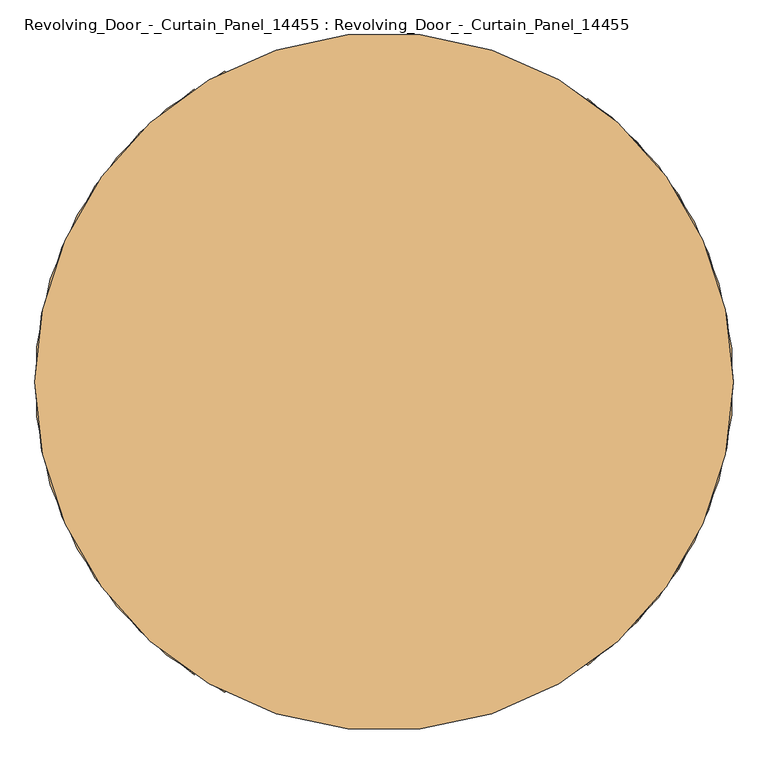
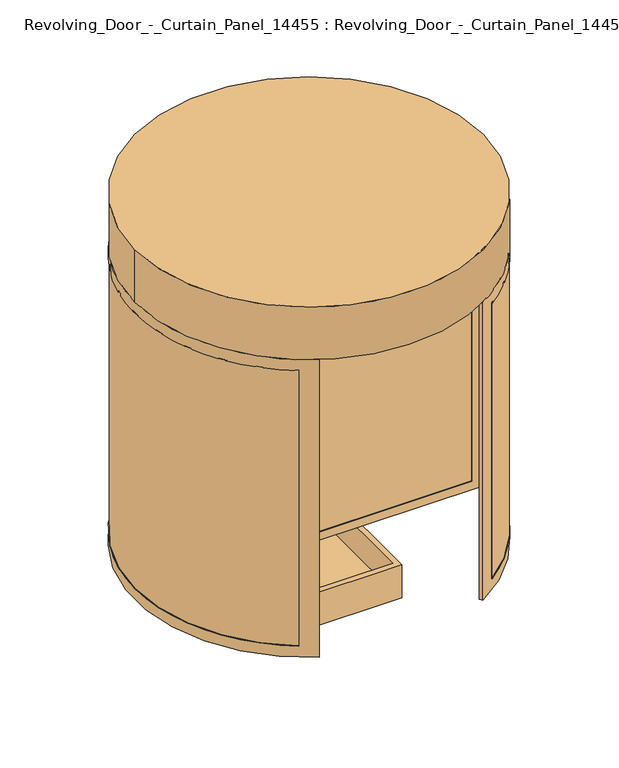
"""IFC4 building model written with IfcOpenShell, lengths in millimetres: door geometry, Revolving_Door_-_Curtain_Panel_14455 : Revolving_Door_-_Curtain_Panel_14455."""

from ifc_helpers import new_model, si_unit, point, frame, origin, origin_with_axes, origin_2d, place, context, project, spatial, polyline, circle_curve, trimmed, segment, composite_curve, outline, extrude, faceted_brep, source, transform, mapped, element, save
from ifc_brep_helpers import plane_surface, cylinder_surface, revolved_surface, advanced_brep


def revolving_door_curtain_panel_14455_revolving_door_curtain_311cc346(model_context):
    return source(origin(), model_context, "Body", "SolidModel", [
        extrude(outline(composite_curve([segment(trimmed(circle_curve(origin_2d(), 1480.0), [point((-804.0011256, -1242.5707988))], [point((-804.0011256, 1242.5707988))], False, "CARTESIAN"), True, "CONTINUOUS"), segment(polyline([(-804.0011256, 1242.5707988), (-793.9880841, 1225.2277022)]), True, "CONTINUOUS"), segment(trimmed(circle_curve(origin_2d(), 1460.0), [point((-793.9880841, 1225.2277022))], [point((-793.9880841, -1225.2277022))], True, "CARTESIAN"), True, "CONTINUOUS"), segment(polyline([(-793.9880841, -1225.2277022), (-804.0011256, -1242.5707988)]), True, "CONTINUOUS")], self_intersect=False)), frame((0.0, 0.0, 100.0), z_axis=(0.0, 0.0, 1.0), x_axis=(1.0, 0.0, 0.0)), (0.0, 0.0, 1.0), 2485.0),
        extrude(outline(composite_curve([segment(polyline([(863.2115619, -1202.1920809), (853.1615488, -1184.7849474)]), True, "CONTINUOUS"), segment(trimmed(circle_curve(origin_2d(), 1460.0), [point((853.1615488, -1184.7849474))], [point((853.1615488, 1184.7849474))], True, "CARTESIAN"), True, "CONTINUOUS"), segment(polyline([(853.1615488, 1184.7849474), (863.2115619, 1202.1920809)]), True, "CONTINUOUS"), segment(trimmed(circle_curve(origin_2d(), 1480.0), [point((863.2115619, 1202.1920809))], [point((863.2115619, -1202.1920809))], False, "CARTESIAN"), True, "CONTINUOUS")], self_intersect=False)), frame((0.0, 0.0, 100.0), z_axis=(0.0, 0.0, 1.0), x_axis=(1.0, 0.0, 0.0)), (0.0, 0.0, 1.0), 2485.0),
        advanced_brep(
        [(-676.6005204, -1321.9064777, 0.0), (-676.6005204, 1321.9064777, 0.0), (-661.580957, 1295.8918309, 0.0), (-661.580957, -1295.8918309, 0.0), (-676.6005204, -1321.9064777, 2685.0), (-661.580957, -1295.8918309, 2685.0), (-661.580957, 1295.8918309, 2685.0), (-791.4847676, 1220.8918309, 2585.0), (-791.4847676, 1220.8918309, 100.0), (-791.4847676, -1220.8918309, 100.0), (-791.4847676, -1220.8918309, 2585.0), (-676.6005204, 1321.9064777, 2685.0), (-806.5043309, -1246.9064777, 2585.0), (-806.5043309, -1246.9064777, 100.0), (-806.5043309, 1246.9064777, 100.0), (-806.5043309, 1246.9064777, 2585.0)],
        [
            (0, 1, circle_curve(frame((0.0, 0.0, 0.0), z_axis=(0.0, 0.0, -1.0), x_axis=(1.0, 0.0, 0.0)), 1485.0)),
            (1, 2),
            (2, 3, circle_curve(origin_with_axes(), 1455.0)),
            (3, 0),
            (4, 0),
            (3, 5),
            (5, 4),
            (2, 6),
            (6, 5, circle_curve(frame((0.0, 0.0, 2685.0), z_axis=(0.0, 0.0, 1.0), x_axis=(1.0, 0.0, 0.0)), 1455.0)),
            (7, 8),
            (8, 9, circle_curve(frame((0.0, 0.0, 100.0), z_axis=(0.0, 0.0, 1.0), x_axis=(1.0, 0.0, 0.0)), 1455.0)),
            (9, 10),
            (10, 7, circle_curve(frame((0.0, 0.0, 2585.0), z_axis=(0.0, 0.0, -1.0), x_axis=(1.0, 0.0, 0.0)), 1455.0)),
            (1, 11),
            (11, 6),
            (4, 11, circle_curve(frame((0.0, 0.0, 2685.0), z_axis=(0.0, 0.0, -1.0), x_axis=(1.0, 0.0, 0.0)), 1485.0)),
            (12, 13),
            (13, 14, circle_curve(frame((0.0, 0.0, 100.0), z_axis=(0.0, 0.0, -1.0), x_axis=(1.0, 0.0, 0.0)), 1485.0)),
            (14, 15),
            (15, 12, circle_curve(frame((0.0, 0.0, 2585.0), z_axis=(0.0, 0.0, 1.0), x_axis=(1.0, 0.0, 0.0)), 1485.0)),
            (14, 8),
            (7, 15),
            (13, 9),
            (12, 10),
        ],
        [
            plane_surface(frame((1485.0, 0.0, 0.0), z_axis=(0.0, 0.0, -1.0), x_axis=(0.0, 1.0, 0.0))),
            plane_surface(frame((-661.580957, -1295.8918309, 2685.0), z_axis=(0.8660254037853362, -0.4999999999984455, 0.0), x_axis=(0.0, 0.0, -1.0))),
            revolved_surface(polyline([(1455.0, 0.0, 0.0), (1455.0, 0.0, 2685.0)]), (0.0, 0.0, 0.0), (0.0, 0.0, -1.0)),
            plane_surface(frame((-676.6005204, 1321.9064777, 2685.0), z_axis=(0.8660254037848054, 0.49999999999936495, 0.0), x_axis=(0.0, 0.0, -1.0))),
            cylinder_surface(origin_with_axes(), 1485.0),
            plane_surface(frame((-806.5043309, 1246.9064777, 2585.0), z_axis=(-0.8660254037848982, -0.4999999999992039, 0.0), x_axis=(0.0, 0.0, -1.0))),
            plane_surface(frame((1485.0, 0.0, 100.0), z_axis=(0.0, 0.0, 1.0), x_axis=(0.0, 1.0, 0.0))),
            plane_surface(frame((-791.4847676, -1220.8918309, 2585.0), z_axis=(-0.8660254037853279, 0.4999999999984598, 0.0), x_axis=(0.0, 0.0, -1.0))),
            plane_surface(frame((1485.0, 0.0, 2685.0), z_axis=(0.0, 0.0, 1.0), x_axis=(0.0, -1.0, 0.0))),
            plane_surface(frame((1485.0, 0.0, 2585.0), z_axis=(0.0, 0.0, -1.0), x_axis=(0.0, -1.0, 0.0))),
        ],
        [
            (0, [[1, 2, 3, 4]]),
            (1, [[5, -4, 6, 7]]),
            (2, [[-6, -3, 8, 9], [10, 11, 12, 13]]),
            (3, [[-8, -2, 14, 15]]),
            (4, [[-14, -1, -5, 16], [17, 18, 19, 20]]),
            (5, [[-19, 21, -10, 22]]),
            (6, [[-18, 23, -11, -21]]),
            (7, [[-12, -23, -17, 24]]),
            (8, [[-7, -9, -15, -16]]),
            (9, [[-20, -22, -13, -24]]),
        ],
    ),
        advanced_brep(
        [(739.4383185, -1287.8105346, 0.0), (724.4382752, -1261.8296975, 0.0), (724.4382752, 1261.8296975, 0.0), (739.4383185, 1287.8105346, 0.0), (739.4383185, -1287.8105346, 2685.0), (739.4383185, 1287.8105346, 2685.0), (865.7238532, 1206.5434969, 2585.0), (865.7238532, 1206.5434969, 100.0), (865.7238532, -1206.5434969, 100.0), (865.7238532, -1206.5434969, 2585.0), (724.4382752, 1261.8296975, 2685.0), (724.4382752, -1261.8296975, 2685.0), (850.648829, -1180.4327892, 2585.0), (850.648829, -1180.4327892, 100.0), (850.648829, 1180.4327892, 100.0), (850.648829, 1180.4327892, 2585.0)],
        [
            (0, 1),
            (1, 2, circle_curve(origin_with_axes(), 1455.0)),
            (2, 3),
            (3, 0, circle_curve(frame((0.0, 0.0, 0.0), z_axis=(0.0, 0.0, -1.0), x_axis=(1.0, 0.0, 0.0)), 1485.0)),
            (4, 0),
            (3, 5),
            (5, 4, circle_curve(frame((0.0, 0.0, 2685.0), z_axis=(0.0, 0.0, -1.0), x_axis=(1.0, 0.0, 0.0)), 1485.0)),
            (6, 7),
            (7, 8, circle_curve(frame((0.0, 0.0, 100.0), z_axis=(0.0, 0.0, -1.0), x_axis=(1.0, 0.0, 0.0)), 1485.0)),
            (8, 9),
            (9, 6, circle_curve(frame((0.0, 0.0, 2585.0), z_axis=(0.0, 0.0, 1.0), x_axis=(1.0, 0.0, 0.0)), 1485.0)),
            (2, 10),
            (10, 5),
            (1, 11),
            (11, 10, circle_curve(frame((0.0, 0.0, 2685.0), z_axis=(0.0, 0.0, 1.0), x_axis=(1.0, 0.0, 0.0)), 1455.0)),
            (12, 13),
            (13, 14, circle_curve(frame((0.0, 0.0, 100.0), z_axis=(0.0, 0.0, 1.0), x_axis=(1.0, 0.0, 0.0)), 1455.0)),
            (14, 15),
            (15, 12, circle_curve(frame((0.0, 0.0, 2585.0), z_axis=(0.0, 0.0, -1.0), x_axis=(1.0, 0.0, 0.0)), 1455.0)),
            (4, 11),
            (7, 14),
            (13, 8),
            (6, 15),
            (12, 9),
        ],
        [
            plane_surface(frame((1485.0, 0.0, 0.0), z_axis=(0.0, 0.0, -1.0), x_axis=(0.0, 1.0, 0.0))),
            cylinder_surface(origin_with_axes(), 1485.0),
            plane_surface(frame((724.4382752, 1261.8296975, 2685.0), z_axis=(-0.866025403784442, 0.49999999999999406, 0.0), x_axis=(0.0, 0.0, -1.0))),
            revolved_surface(polyline([(1455.0, 0.0, 0.0), (1455.0, 0.0, 2685.0)]), (0.0, 0.0, 0.0), (0.0, 0.0, -1.0)),
            plane_surface(frame((739.4383185, -1287.8105346, 2685.0), z_axis=(-0.8660254037846041, -0.49999999999971345, 0.0), x_axis=(0.0, 0.0, -1.0))),
            plane_surface(frame((1485.0, 0.0, 100.0), z_axis=(0.0, 0.0, 1.0), x_axis=(0.0, 1.0, 0.0))),
            plane_surface(frame((850.648829, 1180.4327892, 2585.0), z_axis=(0.8660254037844431, -0.4999999999999923, 0.0), x_axis=(0.0, 0.0, -1.0))),
            plane_surface(frame((865.7238532, -1206.5434969, 2585.0), z_axis=(0.8660254037845999, 0.4999999999997206, 0.0), x_axis=(0.0, 0.0, -1.0))),
            plane_surface(frame((1485.0, 0.0, 2685.0), z_axis=(0.0, 0.0, 1.0), x_axis=(0.0, -1.0, 0.0))),
            plane_surface(frame((1485.0, 0.0, 2585.0), z_axis=(0.0, 0.0, -1.0), x_axis=(0.0, -1.0, 0.0))),
        ],
        [
            (0, [[1, 2, 3, 4]]),
            (1, [[5, -4, 6, 7], [8, 9, 10, 11]]),
            (2, [[-6, -3, 12, 13]]),
            (3, [[-12, -2, 14, 15], [16, 17, 18, 19]]),
            (4, [[-14, -1, -5, 20]]),
            (5, [[-9, 21, -17, 22]]),
            (6, [[-18, -21, -8, 23]]),
            (7, [[-10, -22, -16, 24]]),
            (8, [[-7, -13, -15, -20]]),
            (9, [[-11, -24, -19, -23]]),
        ],
    ),
        extrude(outline(polyline([(-9.9410218, 33.2183548), (-23.7974282, 25.2183548), (-676.2974282, 1155.3815067), (-662.4410218, 1163.3815067), (-9.9410218, 33.2183548)])), frame((0.0, 0.0, 75.0), z_axis=(0.0, 0.0, 1.0), x_axis=(1.0, 0.0, 0.0)), (0.0, 0.0, 1.0), 2535.0),
        extrude(outline(polyline([(1455.0, 0.0), (0.0, 0.0), (0.0, 2685.0), (1455.0, 2685.0), (1455.0, 0.0)]), holes=[polyline([(75.0, 2610.0), (75.0, 75.0), (1380.0, 75.0), (1380.0, 2610.0), (75.0, 2610.0)])]), frame((7.640394, -43.2335505, 0.0), z_axis=(0.8660254037844434, 0.4999999999999919, 0.0), x_axis=(-0.4999999999999919, 0.8660254037844434, 0.0)), (0.0, 0.0, 1.0), 30.0),
        extrude(outline(polyline([(-23.7974282, -25.2183548), (-9.9410218, -33.2183548), (-662.4410218, -1163.3815067), (-676.2974282, -1155.3815067), (-23.7974282, -25.2183548)])), frame((0.0, 0.0, 75.0), z_axis=(0.0, 0.0, 1.0), x_axis=(1.0, 0.0, 0.0)), (0.0, 0.0, 1.0), 2535.0),
        extrude(outline(polyline([(1455.0, 0.0), (0.0, 0.0), (0.0, 2685.0), (1455.0, 2685.0), (1455.0, 0.0)]), holes=[polyline([(75.0, 2610.0), (75.0, 75.0), (1380.0, 75.0), (1380.0, 2610.0), (75.0, 2610.0)])]), frame((33.6211561, 28.2335505, 0.0), z_axis=(-0.8660254037844325, 0.5000000000000107, 0.0), x_axis=(-0.5000000000000107, -0.8660254037844325, 0.0)), (0.0, 0.0, 1.0), 30.0),
        extrude(outline(polyline([(75.0, -8.0), (75.0, 8.0), (1380.0, 8.0), (1380.0, -8.0), (75.0, -8.0)])), frame((0.0, 0.0, 75.0), z_axis=(0.0, 0.0, 1.0), x_axis=(1.0, 0.0, 0.0)), (0.0, 0.0, 1.0), 2535.0),
        extrude(outline(polyline([(0.0, 0.0), (0.0, 1455.0), (2685.0, 1455.0), (2685.0, 0.0), (0.0, 0.0)]), holes=[polyline([(2610.0, 1380.0), (75.0, 1380.0), (75.0, 75.0), (2610.0, 75.0), (2610.0, 1380.0)])]), frame((0.0, -15.0, 0.0), z_axis=(0.0, 1.0, 0.0), x_axis=(0.0, 0.0, 1.0)), (0.0, 0.0, 1.0), 30.0),
        extrude(outline(composite_curve([segment(trimmed(circle_curve(origin_2d(), 50.0), [point((-50.0, 0.0))], [point((50.0, 0.0))], False, "CARTESIAN"), True, "CONTINUOUS"), segment(trimmed(circle_curve(origin_2d(), 50.0), [point((50.0, 0.0))], [point((-50.0, 0.0))], False, "CARTESIAN"), True, "CONTINUOUS")], self_intersect=False)), origin_with_axes(), (0.0, 0.0, 1.0), 2685.0),
        extrude(outline(composite_curve([segment(trimmed(circle_curve(origin_2d(), 1485.0), [point((-1485.0, 0.0))], [point((1485.0, 0.0))], False, "CARTESIAN"), True, "CONTINUOUS"), segment(trimmed(circle_curve(origin_2d(), 1485.0), [point((1485.0, 0.0))], [point((-1485.0, 0.0))], False, "CARTESIAN"), True, "CONTINUOUS")], self_intersect=False)), frame((0.0, 0.0, 2685.0), z_axis=(0.0, 0.0, 1.0), x_axis=(1.0, 0.0, 0.0)), (0.0, 0.0, 1.0), 475.0),
        faceted_brep([(400.0, -542.9342021, -250.0), (400.0, 400.0, -250.0), (-400.0, 400.0, -250.0), (-400.0, -542.9342021, -250.0), (450.0, 450.0, -300.0), (450.0, -592.9342021, -300.0), (-450.0, -592.9342021, -300.0), (-450.0, 450.0, -300.0), (450.0, 450.0, 0.0), (450.0, -592.9342021, 0.0), (-450.0, -592.9342021, 0.0), (-450.0, 450.0, 0.0), (-400.0, -542.9342021, 0.0), (-400.0, 400.0, 0.0), (400.0, 400.0, 0.0), (400.0, -542.9342021, 0.0)], [[[0, 1, 2, 3]], [[4, 5, 6, 7]], [[4, 8, 9, 5]], [[9, 10, 6, 5]], [[10, 11, 7, 6]], [[11, 8, 4, 7]], [[8, 11, 10, 9], [12, 13, 14, 15]], [[15, 0, 3, 12]], [[14, 1, 0, 15]], [[13, 2, 1, 14]], [[12, 3, 2, 13]]]),
    ])


if __name__ == "__main__":
    model = new_model("IFC4")
    model_context = context("Model", 3, world=origin())
    ifc_project = project(units=[si_unit("LENGTHUNIT", "METRE", prefix="MILLI")], contexts=[model_context])
    site = spatial("IfcSite", under=ifc_project)
    building = spatial("IfcBuilding", under=site)
    placement = place(None, origin())
    revolving_door_curtain_panel_14455_revolving_door_curtain_shape = revolving_door_curtain_panel_14455_revolving_door_curtain_311cc346(model_context)
    element("IfcDoor", 1, ObjectType="Revolving_Door_-_Curtain_Panel_14455 : Revolving_Door_-_Curtain_Panel_14455", at=placement, inside=building, context=model_context, shape_type="MappedRepresentation", body=[
        mapped(revolving_door_curtain_panel_14455_revolving_door_curtain_shape, transform((0.0, 0.0, 0.0), x_axis=(1.0, 0.0, 0.0), y_axis=(0.0, 1.0, 0.0), z_axis=(0.0, 0.0, 1.0))),
    ])
    save(model, "model.ifc")

# Revit data of these elements
# Type "Revolving_Door_-_Curtain_Panel_14455 : Revolving_Door_-_Curtain_Panel_14455"
#   Model = "55465463453y7"
#   Manufacturer = "Dublin Doors"
#   Description = "Revolving Door"
#   Type Mark = "42"
#   Fire Rating = "30M"
#   COBie.Type.CreatedBy = "design@eagle.com"
#   COBie.Type.CreatedOn = "2016-09-13T05:47:35"
#   COBie.Type.Name = "Doors_Revolving_Door_-_Curtain_Panel_14455_Revolving_Door_-_Curtain_Panel_14455"
#   COBie.Type.Category = "23-30 10 00 : Doors"
#   COBie.Type.Description = "Revolving Door"
#   COBie.Type.Manufacturer = "Dublin Doors"
#   COBie.Type.ModelNumber = "55465463453y7"
#   Analytic Construction = "<None>"
#   COBie.Type.ReplacementCost = 0
#   Top Cover Thickness = 475 mm
#   Throat Opening [instance default] = 1043 mm
#   Thickness = 1828.8 mm
#   Panel Frame = 75 mm
#   Outer Panel Thickness = 100 mm
#   Outer Glazing OUT = 1480 mm
#   Outer Glazing IN = 1460 mm
#   Middle Post Radius [instance default] = 50 mm
#   Internal Door Clearance [instance default] = 1455 mm
#   Door Radius = 1485 mm
#   COBie.Type = yes
#   Function = 1
#   Pit = none
#   Internal Panels = Metal - Aluminium
#   Glass = Glass, Clear Glazing
#   External Panels = Metal - Aluminium
# Element 1 (IfcDoor, "Revolving_Door_-_Curtain_Panel_14455 : Revolving_Door_-_Curtain_Panel_14455")
#   Materials on its faces: "Metal - Aluminium", "Glass, Clear Glazing"
# Materials
#   "Metal - Aluminium": class "Metal", colour RGB 244 244 244, transparency 0, Cost = 0
#   "Glass, Clear Glazing": class "Glass", colour RGB 0 128 192, transparency 0.75, Description = "Clear glazing", Cost = 0
